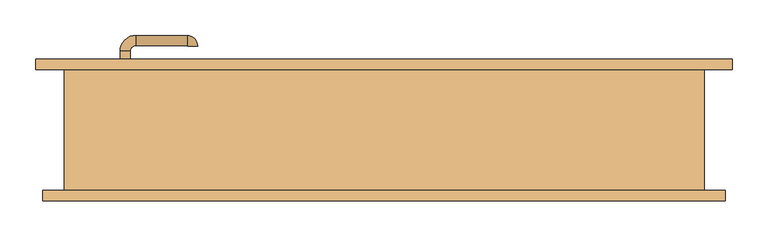
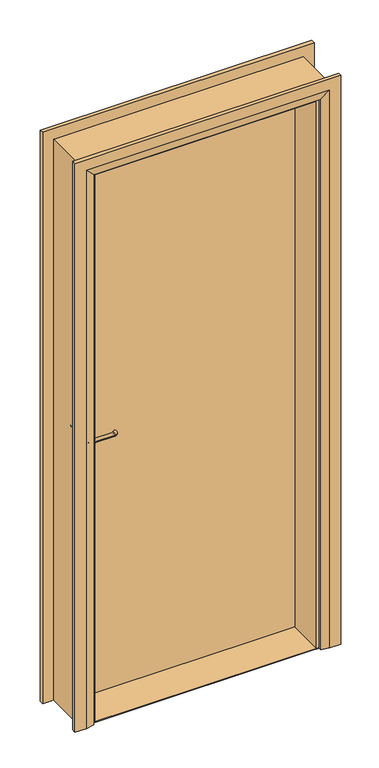
"""IFC4 building model written with IfcOpenShell, lengths in millimetres: door geometry, Porta Simples de Abrir : 80x210cm - Marco de Madeira."""

from ifc_helpers import new_model, si_unit, point, frame, frame_2d, origin, place, context, project, spatial, polyline, circle_curve, ellipse_curve, trimmed, segment, composite_curve, outline, extrude, faceted_brep, source, transform, mapped, element, save
from ifc_brep_helpers import plane_surface, cylinder_surface, revolved_surface, advanced_brep


def door_4ed0e0ed(model_context):
    return source(origin(), model_context, "Body", "SolidModel", [
        extrude(outline(composite_curve([segment(trimmed(circle_curve(frame_2d((1050.0, -364.0)), 20.0), [point((1050.0, -384.0))], [point((1050.0, -344.0))], False, "CARTESIAN"), True, "CONTINUOUS"), segment(trimmed(circle_curve(frame_2d((1050.0, -364.0)), 20.0), [point((1050.0, -344.0))], [point((1050.0, -384.0))], False, "CARTESIAN"), True, "CONTINUOUS")], self_intersect=False)), frame((0.0, 39.4070105, 0.0), z_axis=(0.0, 1.0, 0.0), x_axis=(0.0, 0.0, 1.0)), (0.0, 0.0, 1.0), 4.5929895),
        advanced_brep(
        [(-357.0, 39.4070105, 1050.0), (-371.0, 39.4070105, 1050.0), (-371.0, 24.0, 1050.0), (-357.0, 24.0, 1050.0), (-349.0, 2.0, 1050.0), (-349.0, 16.0, 1050.0), (-277.0, 2.0, 1050.0), (-277.0, 16.0, 1050.0), (-276.0, 17.0, 1050.0), (-262.0, 17.0, 1050.0)],
        [
            (0, 1, circle_curve(frame((-364.0, 39.4070105, 1050.0), z_axis=(0.0, 1.0, 0.0), x_axis=(-1.0, 0.0, 0.0)), 7.0)),
            (1, 0, circle_curve(frame((-364.0, 39.4070105, 1050.0), z_axis=(0.0, 1.0, 0.0), x_axis=(-1.0, 0.0, 0.0)), 7.0)),
            (1, 2),
            (2, 3, circle_curve(frame((-364.0, 24.0, 1050.0), z_axis=(0.0, 1.0, 0.0), x_axis=(-1.0, 0.0, 0.0)), 7.0)),
            (3, 0),
            (3, 2, circle_curve(frame((-364.0, 24.0, 1050.0), z_axis=(0.0, 1.0, 0.0), x_axis=(-1.0, 0.0, 0.0)), 7.0)),
            (4, 5, circle_curve(frame((-349.0, 9.0, 1050.0), z_axis=(-1.0, 0.0, 0.0), x_axis=(0.0, -1.0, 0.0)), 7.0)),
            (5, 3, circle_curve(frame((-349.0, 24.0, 1050.0), z_axis=(0.0, 0.0, -1.0), x_axis=(-1.0, 0.0, 0.0)), 8.0)),
            (2, 4, circle_curve(frame((-349.0, 24.0, 1050.0), z_axis=(0.0, 0.0, 1.0), x_axis=(-1.0, 0.0, 0.0)), 22.0)),
            (5, 4, circle_curve(frame((-349.0, 9.0, 1050.0), z_axis=(-1.0, 0.0, 0.0), x_axis=(0.0, -1.0, 0.0)), 7.0)),
            (4, 6),
            (6, 7, circle_curve(frame((-277.0, 9.0, 1050.0), z_axis=(-1.0, 0.0, 0.0), x_axis=(0.0, -1.0, 0.0)), 7.0)),
            (7, 5),
            (7, 6, circle_curve(frame((-277.0, 9.0, 1050.0), z_axis=(-1.0, 0.0, 0.0), x_axis=(0.0, -1.0, 0.0)), 7.0)),
            (8, 9, circle_curve(frame((-269.0, 17.0, 1050.0), z_axis=(0.0, 1.0, 0.0), x_axis=(1.0, 0.0, 0.0)), 7.0)),
            (9, 8, circle_curve(frame((-269.0, 17.0, 1050.0), z_axis=(0.0, 1.0, 0.0), x_axis=(1.0, 0.0, 0.0)), 7.0)),
            (8, 7, circle_curve(frame((-277.0, 17.0, 1050.0), z_axis=(0.0, 0.0, -1.0), x_axis=(0.0, -1.0, 0.0)), 1.0)),
            (6, 9, circle_curve(frame((-277.0, 17.0, 1050.0), z_axis=(0.0, 0.0, 1.0), x_axis=(0.0, -1.0, 0.0)), 15.0)),
        ],
        [
            plane_surface(frame((-364.0, 39.4070105, 1050.0), z_axis=(0.0, 1.0, 0.0), x_axis=(0.0, 0.0, 1.0))),
            cylinder_surface(frame((-364.0, 39.4070105, 1050.0), z_axis=(0.0, 1.0, 0.0), x_axis=(-1.0, 0.0, 0.0)), 7.0),
            revolved_surface(trimmed(ellipse_curve(frame((-364.0, 24.0, 1050.0), z_axis=(0.0, -1.0, 0.0), x_axis=(-1.0, 0.0, 0.0)), 7.0, 7.0), [point((-357.0, 24.0, 1050.0))], [point((-371.0, 24.0, 1050.0))], True, "CARTESIAN"), (-349.0, 24.0, 1050.0), (0.0, 0.0, -1.0)),
            revolved_surface(trimmed(ellipse_curve(frame((-364.0, 24.0, 1050.0), z_axis=(0.0, -1.0, 0.0), x_axis=(-1.0, 0.0, 0.0)), 7.0, 7.0), [point((-371.0, 24.0, 1050.0))], [point((-357.0, 24.0, 1050.0))], True, "CARTESIAN"), (-349.0, 24.0, 1050.0), (0.0, 0.0, -1.0)),
            cylinder_surface(frame((-349.0, 9.0, 1050.0), z_axis=(-1.0, 0.0, 0.0), x_axis=(0.0, -1.0, 0.0)), 7.0),
            plane_surface(frame((-269.0, 17.0, 1050.0), z_axis=(0.0, 1.0, 0.0), x_axis=(0.0, 0.0, 1.0))),
            revolved_surface(trimmed(ellipse_curve(frame((-277.0, 9.0, 1050.0), z_axis=(1.0, 0.0, 0.0), x_axis=(0.0, -1.0, 0.0)), 7.0, 7.0), [point((-277.0, 16.0, 1050.0))], [point((-277.0, 2.0, 1050.0))], True, "CARTESIAN"), (-277.0, 17.0, 1050.0), (0.0, 0.0, -1.0)),
            revolved_surface(trimmed(ellipse_curve(frame((-277.0, 9.0, 1050.0), z_axis=(1.0, 0.0, 0.0), x_axis=(0.0, -1.0, 0.0)), 7.0, 7.0), [point((-277.0, 2.0, 1050.0))], [point((-277.0, 16.0, 1050.0))], True, "CARTESIAN"), (-277.0, 17.0, 1050.0), (0.0, 0.0, -1.0)),
        ],
        [
            (0, [[1, 2]]),
            (1, [[3, 4, 5, -2]]),
            (1, [[-5, 6, -3, -1]]),
            (2, [[7, 8, -4, 9]]),
            (3, [[10, -9, -6, -8]]),
            (4, [[11, 12, 13, -7]]),
            (4, [[-13, 14, -11, -10]]),
            (5, [[15, 16]]),
            (6, [[-15, 17, -12, 18]]),
            (7, [[-16, -18, -14, -17]]),
        ],
    ),
        extrude(outline(polyline([(-334.0, 50.0), (-334.0, 44.0), (-394.0, 44.0), (-394.0, 50.0), (-334.0, 50.0)])), frame((0.0, 0.0, 925.0), z_axis=(0.0, 0.0, 1.0), x_axis=(1.0, 0.0, 0.0)), (0.0, 0.0, 1.0), 165.0),
        extrude(outline(composite_curve([segment(trimmed(circle_curve(frame_2d((1050.0, -364.0)), 20.0), [point((1050.0, -384.0))], [point((1050.0, -344.0))], False, "CARTESIAN"), True, "CONTINUOUS"), segment(trimmed(circle_curve(frame_2d((1050.0, -364.0)), 20.0), [point((1050.0, -344.0))], [point((1050.0, -384.0))], False, "CARTESIAN"), True, "CONTINUOUS")], self_intersect=False)), frame((0.0, 91.0, 0.0), z_axis=(0.0, 1.0, 0.0), x_axis=(0.0, 0.0, 1.0)), (0.0, 0.0, 1.0), 4.5929895),
        advanced_brep(
        [(-357.0, 95.5929895, 1050.0), (-371.0, 95.5929895, 1050.0), (-357.0, 111.0, 1050.0), (-371.0, 111.0, 1050.0), (-349.0, 133.0, 1050.0), (-349.0, 119.0, 1050.0), (-277.0, 119.0, 1050.0), (-277.0, 133.0, 1050.0), (-276.0, 118.0, 1050.0), (-262.0, 118.0, 1050.0)],
        [
            (0, 1, circle_curve(frame((-364.0, 95.5929895, 1050.0), z_axis=(0.0, -1.0, 0.0), x_axis=(-1.0, 0.0, 0.0)), 7.0)),
            (1, 0, circle_curve(frame((-364.0, 95.5929895, 1050.0), z_axis=(0.0, -1.0, 0.0), x_axis=(-1.0, 0.0, 0.0)), 7.0)),
            (0, 2),
            (2, 3, circle_curve(frame((-364.0, 111.0, 1050.0), z_axis=(0.0, -1.0, 0.0), x_axis=(-1.0, 0.0, 0.0)), 7.0)),
            (3, 1),
            (3, 2, circle_curve(frame((-364.0, 111.0, 1050.0), z_axis=(0.0, -1.0, 0.0), x_axis=(-1.0, 0.0, 0.0)), 7.0)),
            (4, 3, circle_curve(frame((-349.0, 111.0, 1050.0), z_axis=(0.0, 0.0, 1.0), x_axis=(-1.0, 0.0, 0.0)), 22.0)),
            (2, 5, circle_curve(frame((-349.0, 111.0, 1050.0), z_axis=(0.0, 0.0, -1.0), x_axis=(-1.0, 0.0, 0.0)), 8.0)),
            (5, 4, circle_curve(frame((-349.0, 126.0, 1050.0), z_axis=(-1.0, 0.0, 0.0), x_axis=(0.0, 1.0, 0.0)), 7.0)),
            (4, 5, circle_curve(frame((-349.0, 126.0, 1050.0), z_axis=(-1.0, 0.0, 0.0), x_axis=(0.0, 1.0, 0.0)), 7.0)),
            (5, 6),
            (6, 7, circle_curve(frame((-277.0, 126.0, 1050.0), z_axis=(-1.0, 0.0, 0.0), x_axis=(0.0, 1.0, 0.0)), 7.0)),
            (7, 4),
            (7, 6, circle_curve(frame((-277.0, 126.0, 1050.0), z_axis=(-1.0, 0.0, 0.0), x_axis=(0.0, 1.0, 0.0)), 7.0)),
            (8, 9, circle_curve(frame((-269.0, 118.0, 1050.0), z_axis=(0.0, -1.0, 0.0), x_axis=(1.0, 0.0, 0.0)), 7.0)),
            (9, 8, circle_curve(frame((-269.0, 118.0, 1050.0), z_axis=(0.0, -1.0, 0.0), x_axis=(1.0, 0.0, 0.0)), 7.0)),
            (9, 7, circle_curve(frame((-277.0, 118.0, 1050.0), z_axis=(0.0, 0.0, 1.0), x_axis=(0.0, 1.0, 0.0)), 15.0)),
            (6, 8, circle_curve(frame((-277.0, 118.0, 1050.0), z_axis=(0.0, 0.0, -1.0), x_axis=(0.0, 1.0, 0.0)), 1.0)),
        ],
        [
            plane_surface(frame((-364.0, 95.5929895, 1050.0), z_axis=(0.0, -1.0, 0.0), x_axis=(0.0, 0.0, 1.0))),
            cylinder_surface(frame((-364.0, 95.5929895, 1050.0), z_axis=(0.0, -1.0, 0.0), x_axis=(-1.0, 0.0, 0.0)), 7.0),
            revolved_surface(trimmed(ellipse_curve(frame((-364.0, 111.0, 1050.0), z_axis=(0.0, -1.0, 0.0), x_axis=(-1.0, 0.0, 0.0)), 7.0, 7.0), [point((-357.0, 111.0, 1050.0))], [point((-371.0, 111.0, 1050.0))], True, "CARTESIAN"), (-349.0, 111.0, 1050.0), (0.0, 0.0, -1.0)),
            revolved_surface(trimmed(ellipse_curve(frame((-364.0, 111.0, 1050.0), z_axis=(0.0, -1.0, 0.0), x_axis=(-1.0, 0.0, 0.0)), 7.0, 7.0), [point((-371.0, 111.0, 1050.0))], [point((-357.0, 111.0, 1050.0))], True, "CARTESIAN"), (-349.0, 111.0, 1050.0), (0.0, 0.0, -1.0)),
            cylinder_surface(frame((-349.0, 126.0, 1050.0), z_axis=(-1.0, 0.0, 0.0), x_axis=(0.0, 1.0, 0.0)), 7.0),
            plane_surface(frame((-269.0, 118.0, 1050.0), z_axis=(0.0, -1.0, 0.0), x_axis=(0.0, 0.0, 1.0))),
            revolved_surface(trimmed(ellipse_curve(frame((-277.0, 126.0, 1050.0), z_axis=(-1.0, 0.0, 0.0), x_axis=(0.0, 1.0, 0.0)), 7.0, 7.0), [point((-277.0, 119.0, 1050.0))], [point((-277.0, 133.0, 1050.0))], True, "CARTESIAN"), (-277.0, 118.0, 1050.0), (0.0, 0.0, -1.0)),
            revolved_surface(trimmed(ellipse_curve(frame((-277.0, 126.0, 1050.0), z_axis=(-1.0, 0.0, 0.0), x_axis=(0.0, 1.0, 0.0)), 7.0, 7.0), [point((-277.0, 133.0, 1050.0))], [point((-277.0, 119.0, 1050.0))], True, "CARTESIAN"), (-277.0, 118.0, 1050.0), (0.0, 0.0, -1.0)),
        ],
        [
            (0, [[1, 2]]),
            (1, [[-1, 3, 4, 5]]),
            (1, [[-2, -5, 6, -3]]),
            (2, [[7, -4, 8, 9]]),
            (3, [[-8, -6, -7, 10]]),
            (4, [[-9, 11, 12, 13]]),
            (4, [[-10, -13, 14, -11]]),
            (5, [[15, 16]]),
            (6, [[17, -12, 18, -16]]),
            (7, [[-18, -14, -17, -15]]),
        ],
    ),
        extrude(outline(polyline([(-334.0, 85.0), (-394.0, 85.0), (-394.0, 91.0), (-334.0, 91.0), (-334.0, 85.0)])), frame((0.0, 0.0, 925.0), z_axis=(0.0, 0.0, 1.0), x_axis=(1.0, 0.0, 0.0)), (0.0, 0.0, 1.0), 165.0),
        extrude(outline(polyline([(408.0, 50.0), (-408.0, 50.0), (-408.0, 85.0), (408.0, 85.0), (408.0, 50.0)])), frame((0.0, 0.0, 53.0), z_axis=(0.0, 0.0, 1.0), x_axis=(1.0, 0.0, 0.0)), (0.0, 0.0, 1.0), 2094.0),
        faceted_brep([(480.0, -85.0, 50.0), (480.0, -100.0, 50.0), (440.0, -100.0, 50.0), (410.0, -95.0, 50.0), (410.0, -85.0, 50.0), (480.0, -85.0, 2220.0), (480.0, -100.0, 2220.0), (-480.0, -100.0, 2220.0), (-480.0, -100.0, 50.0), (-440.0, -100.0, 50.0), (-440.0, -100.0, 2180.0), (440.0, -100.0, 2180.0), (410.0, -95.0, 2150.0), (410.0, -85.0, 2150.0), (-410.0, -85.0, 2150.0), (-410.0, -85.0, 50.0), (-480.0, -85.0, 50.0), (-480.0, -85.0, 2220.0), (-410.0, -95.0, 2150.0), (-410.0, -95.0, 50.0)], [[[0, 1, 2, 3, 4]], [[1, 0, 5, 6]], [[2, 1, 6, 7, 8, 9, 10, 11]], [[3, 2, 11, 12]], [[4, 3, 12, 13]], [[0, 4, 13, 14, 15, 16, 17, 5]], [[14, 18, 19, 15]], [[16, 15, 19, 9, 8]], [[7, 17, 16, 8]], [[18, 10, 9, 19]], [[13, 12, 18, 14]], [[6, 5, 17, 7]], [[12, 11, 10, 18]]]),
        faceted_brep([(490.0, 85.0, 50.0), (420.0, 85.0, 50.0), (420.0, 95.0, 50.0), (450.0, 100.0, 50.0), (490.0, 100.0, 50.0), (490.0, 85.0, 2230.0), (-490.0, 85.0, 2230.0), (-490.0, 85.0, 50.0), (-420.0, 85.0, 50.0), (-420.0, 85.0, 2160.0), (420.0, 85.0, 2160.0), (420.0, 95.0, 2160.0), (450.0, 100.0, 2190.0), (-450.0, 100.0, 2190.0), (-450.0, 100.0, 50.0), (-490.0, 100.0, 50.0), (-490.0, 100.0, 2230.0), (490.0, 100.0, 2230.0), (-420.0, 95.0, 50.0), (-420.0, 95.0, 2160.0)], [[[0, 1, 2, 3, 4]], [[1, 0, 5, 6, 7, 8, 9, 10]], [[2, 1, 10, 11]], [[3, 2, 11, 12]], [[4, 3, 12, 13, 14, 15, 16, 17]], [[0, 4, 17, 5]], [[6, 16, 15, 7]], [[7, 15, 14, 18, 8]], [[19, 9, 8, 18]], [[13, 19, 18, 14]], [[11, 10, 9, 19]], [[5, 17, 16, 6]], [[12, 11, 19, 13]]]),
        faceted_brep([(-410.0, 85.0, 50.0), (-410.0, 48.0, 50.0), (-400.0, 48.0, 50.0), (-400.0, -85.0, 50.0), (-450.0, -85.0, 50.0), (-450.0, 85.0, 50.0), (-410.0, 85.0, 2150.0), (-410.0, 48.0, 2150.0), (-400.0, 48.0, 2140.0), (-400.0, -85.0, 2140.0), (-450.0, -85.0, 2190.0), (-450.0, 85.0, 2190.0), (410.0, 85.0, 50.0), (450.0, 85.0, 50.0), (450.0, -85.0, 50.0), (400.0, -85.0, 50.0), (400.0, 48.0, 50.0), (410.0, 48.0, 50.0), (410.0, 85.0, 2150.0), (450.0, 85.0, 2190.0), (450.0, -85.0, 2190.0), (400.0, -85.0, 2140.0), (400.0, 48.0, 2140.0), (410.0, 48.0, 2150.0)], [[[0, 1, 2, 3, 4, 5]], [[1, 0, 6, 7]], [[2, 1, 7, 8]], [[3, 2, 8, 9]], [[4, 3, 9, 10]], [[5, 4, 10, 11]], [[0, 5, 11, 6]], [[12, 13, 14, 15, 16, 17]], [[18, 19, 13, 12]], [[19, 20, 14, 13]], [[20, 21, 15, 14]], [[21, 22, 16, 15]], [[22, 23, 17, 16]], [[23, 18, 12, 17]], [[7, 6, 18, 23]], [[8, 7, 23, 22]], [[9, 8, 22, 21]], [[10, 9, 21, 20]], [[11, 10, 20, 19]], [[6, 11, 19, 18]]]),
        extrude(outline(polyline([(450.0, 50.0), (450.0, -85.0), (-450.0, -85.0), (-450.0, 50.0), (450.0, 50.0)])), frame((0.0, 0.0, 50.0), z_axis=(0.0, 0.0, 1.0), x_axis=(1.0, 0.0, 0.0)), (0.0, 0.0, 1.0), 3.0),
    ])


if __name__ == "__main__":
    model = new_model("IFC4")
    model_context = context("Model", 3, world=origin())
    ifc_project = project(units=[si_unit("LENGTHUNIT", "METRE", prefix="MILLI")], contexts=[model_context])
    site = spatial("IfcSite", under=ifc_project)
    building = spatial("IfcBuilding", under=site)
    placement = place(None, origin())
    door_shape = door_4ed0e0ed(model_context)
    element("IfcDoor", 1, ObjectType="Porta Simples de Abrir : 80x210cm - Marco de Madeira", at=placement, inside=building, context=model_context, shape_type="MappedRepresentation", body=[
        mapped(door_shape, transform((0.0, 0.0, 0.0), x_axis=(1.0, 0.0, 0.0), y_axis=(0.0, 1.0, 0.0), z_axis=(0.0, 0.0, 1.0))),
    ])
    save(model, "model.ifc")

# Revit data of these elements
# Type "Porta Simples de Abrir : 80x210cm - Marco de Madeira"
#   Type Mark = "P57"
#   SINAPI = ""
#   Analytic Construction = "<Nenhum>"
#   Construction Type = "300"
#   Maçaneta [instance default] = ""
#   Fechadura [instance default] = ""
#   Vão Luz (somente para informação) = 0.780 m
#   Tolerância Folha Vertical = 0.003 m
#   Módulo Básico M = 0.100 m
#   Largura de Coordenação Modular Largura CM = 0.900 m
#   Rough Width = 0.900 m
#   Deslocamento da Horizontal da Folha = 0.000 m
#   Altura de Coordenação Modular Largura CM = 2.200 m
#   Rough Height = 2.200 m
#   Altura Nominal = 2.090 m
#   Ajuste de Coordenação Topo AC Topo = 0.010 m
#   Ajuste de Coordenação Base AC Base = 0.050 m
#   Ajuste de Coordenação AC = 0.010 m
#   Tolerância Folha Horizontal = 0.002 m
#   Largura Folha (somente para informação) = 0.796 m
#   Espessura Folha = 0.035 m
#   Maçaneta - Distância da Folha = 0.044 m
#   Maçaneta - Altura = 1.000 m
#   Largura Nominal (Largura Mn) = 0.820 m
#   Distância do Nível = 0.003 m
#   Aduela Interna Espessura = 0.040 m
#   Aduela Externa Espessura = 0.050 m
#   Altura Folha (somente para informação) = 2.075 m
#   Height = 2.140 m
#   Width = 0.880 m
#   Número de Módulos Básicos nM Largura = 9
#   Número de Módulos Básicos nM Altura = 22
#   Marco Metálico = no
#   Aduela de Madeira = no
#   Aduela Metálica de Canto = no
#   Guarnição Reta = no
#   Guarnição Chanfrada = yes
#   Batente - Material [instance default] = none
#   Painel - Material [instance default] = none
#   Model = ""
#   Function = (empty or 0)
#   Description = (empty or 0)
#   Wall Closure = (empty or 0)
#   Assembly Code = ""
# Element 1 (IfcDoor, "Porta Simples de Abrir : 80x210cm - Marco de Madeira")
#   Materials on its faces: "Porta - Maçaneta", "GRANITO"
# Materials
#   "Porta - Maçaneta": class "Diversos", colour RGB 0 0 0, transparency 0
#   "GRANITO": class "Genérico", colour RGB 120 120 120, transparency 0, Cost = 0
